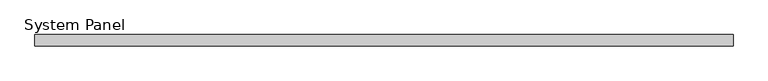
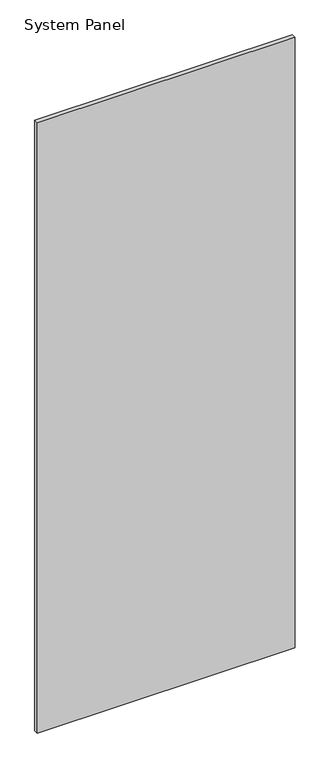
"""IFC4 building model written with IfcOpenShell, lengths in millimetres: plate geometry, System Panel : WWm-Glass-20mm-10mmOffset."""

from ifc_helpers import new_model, si_unit, origin, origin_with_axes, place, context, project, spatial, polyline, outline, extrude, source, transform, mapped, element, save


def system_panel_59bcb82b(model_context):
    return source(origin(), model_context, "Body", "SweptSolid", [
        extrude(outline(polyline([(629.1992668, 0.0), (-629.1992668, 0.0), (-629.1992668, 20.0), (629.1992668, 20.0), (629.1992668, 0.0)])), origin_with_axes(), (0.0, 0.0, 1.0), 3150.0),
    ])


if __name__ == "__main__":
    model = new_model("IFC4")
    model_context = context("Model", 3, world=origin())
    ifc_project = project(units=[si_unit("LENGTHUNIT", "METRE", prefix="MILLI")], contexts=[model_context])
    site = spatial("IfcSite", under=ifc_project)
    building = spatial("IfcBuilding", under=site)
    placement = place(None, origin())
    system_panel_shape = system_panel_59bcb82b(model_context)
    element("IfcPlate", 1, ObjectType="System Panel : WWm-Glass-20mm-10mmOffset", at=placement, inside=building, context=model_context, shape_type="MappedRepresentation", body=[
        mapped(system_panel_shape, transform((0.0, 0.0, 0.0), x_axis=(1.0, 0.0, 0.0), y_axis=(0.0, 1.0, 0.0), z_axis=(0.0, 0.0, 1.0))),
    ])
    save(model, "model.ifc")

# Revit data of these elements
# Type "System Panel : WWm-Glass-20mm-10mmOffset"
#   Finish = ""
# Element 1 (IfcPlate, "System Panel : WWm-Glass-20mm-10mmOffset")
#   Materials on its faces: "WW-EC-GL-Storefront"
# Materials
#   "WW-EC-GL-Storefront": class "Glass", colour RGB 236 240 239, transparency 0.85, Description = "Storefront Glass", Cost = 0
